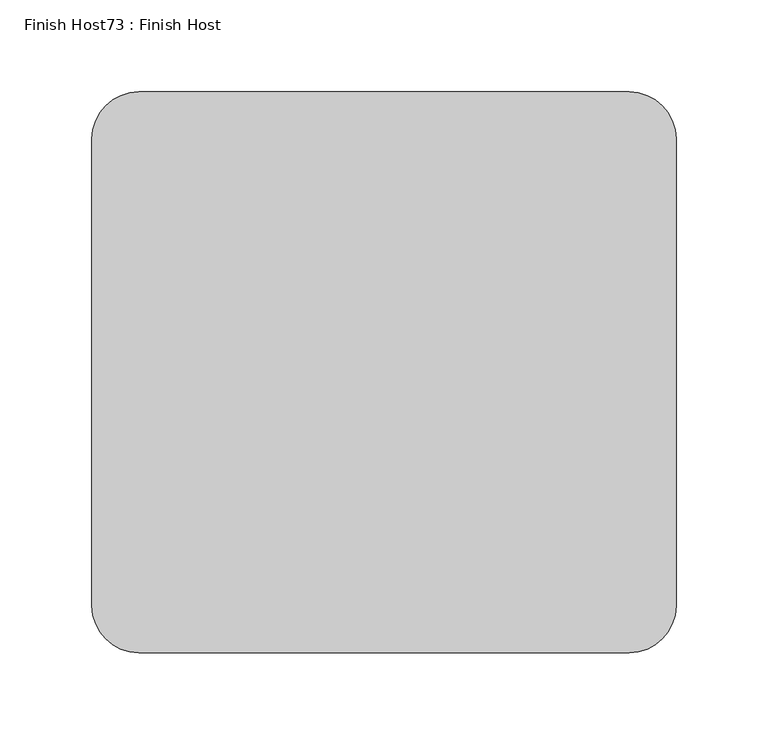
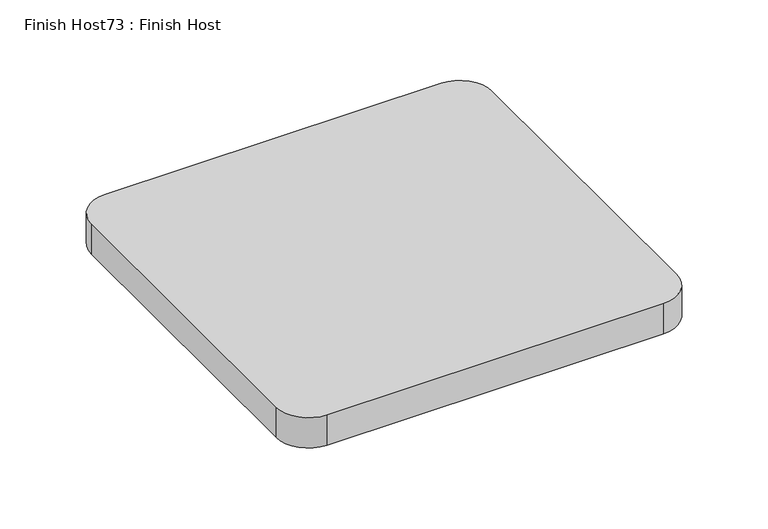
"""IFC4 building model written with IfcOpenShell, lengths in millimetres: proxy geometry, Finish Host73 : Finish Host."""

from ifc_helpers import new_model, si_unit, point, frame_2d, origin, origin_with_axes, place, context, project, spatial, polyline, circle_curve, trimmed, segment, composite_curve, outline, extrude, source, transform, mapped, element, save


def finish_host73_finish_host_d23a8eab(model_context):
    return source(origin(), model_context, "Body", "SweptSolid", [
        extrude(outline(composite_curve([segment(polyline([(-17114.188729, 1376.6189424), (-17114.188729, 1630.6189424)]), True, "CONTINUOUS"), segment(trimmed(circle_curve(frame_2d((-17088.788729, 1630.6189424)), 25.4), [point((-17114.188729, 1630.6189424))], [point((-17088.788729, 1656.0189424))], False, "CARTESIAN"), True, "CONTINUOUS"), segment(polyline([(-17088.788729, 1656.0189424), (-16822.088729, 1656.0189424)]), True, "CONTINUOUS"), segment(trimmed(circle_curve(frame_2d((-16822.088729, 1630.6189424)), 25.4), [point((-16822.088729, 1656.0189424))], [point((-16796.688729, 1630.6189424))], False, "CARTESIAN"), True, "CONTINUOUS"), segment(polyline([(-16796.688729, 1630.6189424), (-16796.688729, 1376.6189424)]), True, "CONTINUOUS"), segment(trimmed(circle_curve(frame_2d((-16822.088729, 1376.6189424)), 25.4), [point((-16796.688729, 1376.6189424))], [point((-16822.088729, 1351.2189424))], False, "CARTESIAN"), True, "CONTINUOUS"), segment(polyline([(-16822.088729, 1351.2189424), (-17088.788729, 1351.2189424)]), True, "CONTINUOUS"), segment(trimmed(circle_curve(frame_2d((-17088.788729, 1376.6189424)), 25.4), [point((-17088.788729, 1351.2189424))], [point((-17114.188729, 1376.6189424))], False, "CARTESIAN"), True, "CONTINUOUS")], self_intersect=False)), origin_with_axes(), (0.0, 0.0, 1.0), 25.4),
    ])


if __name__ == "__main__":
    model = new_model("IFC4")
    model_context = context("Model", 3, world=origin())
    ifc_project = project(units=[si_unit("LENGTHUNIT", "METRE", prefix="MILLI")], contexts=[model_context])
    site = spatial("IfcSite", under=ifc_project)
    building = spatial("IfcBuilding", under=site)
    placement = place(None, origin())
    finish_host73_finish_host_shape = finish_host73_finish_host_d23a8eab(model_context)
    element("IfcBuildingElementProxy", 1, Name="Finish Host73 : Finish Host", ObjectType="Finish Host73 : Finish Host", at=placement, inside=building, context=model_context, shape_type="MappedRepresentation", body=[
        mapped(finish_host73_finish_host_shape, transform((0.0, 0.0, 0.0), x_axis=(1.0, 0.0, 0.0), y_axis=(0.0, 1.0, 0.0), z_axis=(0.0, 0.0, 1.0))),
    ])
    save(model, "model.ifc")

# Revit data of these elements
# Type "Finish Host73 : Finish Host"
#   Countertop Material = Stone - Teknion - MQ - White Carrera
# Element 1 (IfcBuildingElementProxy, "Finish Host73 : Finish Host")
#   Materials on its faces: "Stone - Teknion - MQ - White Carrera"
# Materials
#   "Stone - Teknion - MQ - White Carrera": class "Metal", colour RGB 142 141 140, transparency 0, Model = "MQ G", Manufacturer = "Teknion Studio", URL = "http://www.teknion.com/", Description = "White Carrera Marble", Cost = 0
